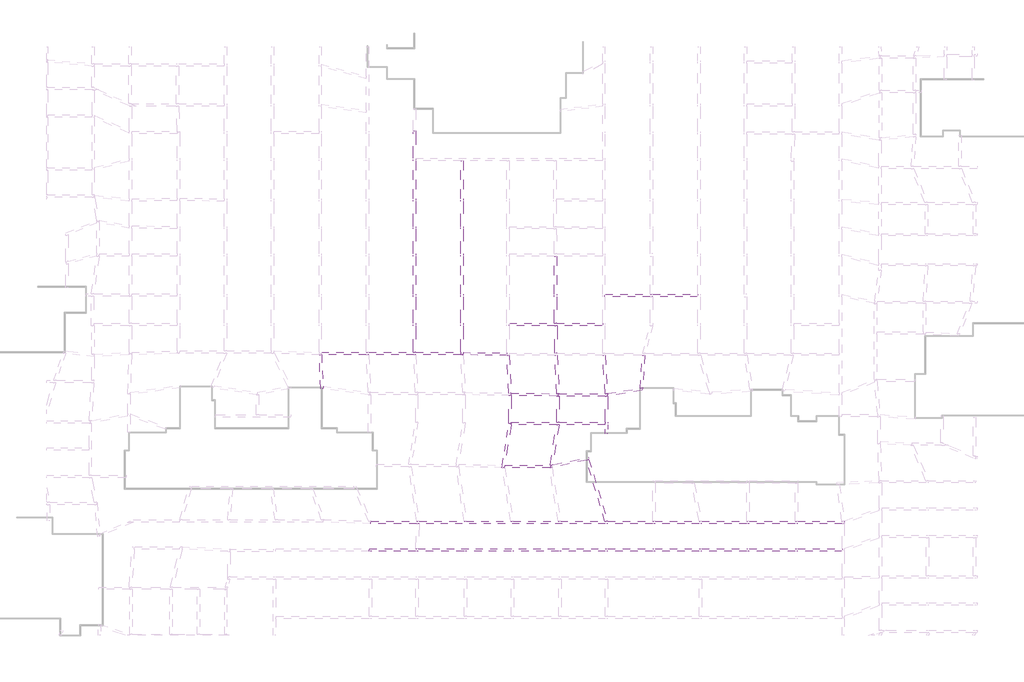
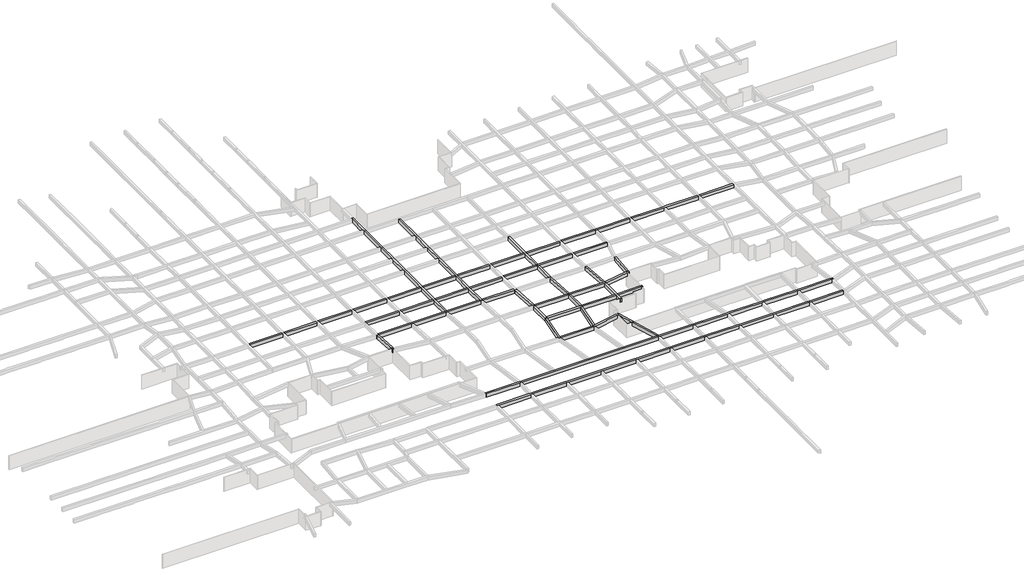
# One storey, part 21 of 45: 27 beams.
"""IFC4 building model written with IfcOpenShell, lengths in millimetres."""

from ifc_helpers import new_model, si_unit, frame, origin, place, context, project, spatial, polyline, outline, extrude, faceted_brep, element, save

model = new_model("IFC4")

# Units and contexts
model_context = context("Model", 3, world=origin())
ifc_project = project(units=[si_unit("LENGTHUNIT", "METRE", prefix="MILLI")], contexts=[model_context])

# Site, building, storey
site = spatial("IfcSite", under=ifc_project)
building = spatial("IfcBuilding", under=site)
storey = spatial("IfcBuildingStorey", under=building, Name="户型图", Elevation=0.0)

# Beams
placement = place(None, origin())
element("IfcBeam", 1, ObjectType="混凝土 - 矩形梁 : KL_beam", at=placement, inside=storey, context=model_context, shape_type="Brep", body=[
    faceted_brep([(-45810.5958048, 7704.0007632, 3300.0), (-45411.0008038, 7704.0007632, 3300.0), (-45410.5958048, 7704.0007632, 3300.0), (-45410.5958048, 7704.0007632, 2500.0), (-45411.0008038, 7704.0007632, 2500.0), (-45810.5958048, 7704.0007632, 2500.0), (-45810.5958048, 7600.318112, 3300.0), (-45810.5958048, 7200.318112, 3300.0), (-45810.5958048, 3119.5822838, 3300.0), (-45810.5958048, 2719.5822838, 3300.0), (-45810.5958048, -3551.5199121, 3300.0), (-45810.5958048, -3951.5199121, 3300.0), (-45810.5958048, -8106.533538, 3300.0), (-45810.5958048, -8506.533538, 3300.0), (-45810.5958048, -12606.533538, 3300.0), (-45810.5958048, -13006.533538, 3300.0), (-45810.5958048, -19266.2432363, 3300.0), (-45810.5958048, -19666.2432363, 3300.0), (-45810.5958048, -24066.2432363, 3300.0), (-45810.5958048, -24466.2432363, 3300.0), (-45810.5958048, -28866.2296815, 3300.0), (-45410.5958048, -28866.2296815, 3300.0), (-45410.5958048, -24466.2432363, 3300.0), (-45410.5958048, -24066.2432363, 3300.0), (-45410.5958048, -19666.2432363, 3300.0), (-45410.5958048, -19266.2432363, 3300.0), (-45410.5958048, -13006.533538, 3300.0), (-45410.5958048, -12606.533538, 3300.0), (-45410.5958048, -8506.533538, 3300.0), (-45410.5958048, -8106.533538, 3300.0), (-45410.5958048, -3951.5199121, 3300.0), (-45410.5958048, -3551.5199121, 3300.0), (-45410.5958048, 2719.5822838, 3300.0), (-45410.5958048, 3119.5822838, 3300.0), (-45410.5958048, -28866.2296815, 2500.0), (-45410.5958048, -24466.2432363, 2500.0), (-45410.5958048, -24066.2432363, 2500.0), (-45410.5958048, -19666.2432363, 2500.0), (-45410.5958048, -19266.2432363, 2500.0), (-45410.5958048, -13006.533538, 2500.0), (-45410.5958048, -12606.533538, 2500.0), (-45410.5958048, -8506.533538, 2500.0), (-45410.5958048, -8106.533538, 2500.0), (-45410.5958048, -3951.5199121, 2500.0), (-45410.5958048, -3551.5199121, 2500.0), (-45410.5958048, 2719.5822838, 2500.0), (-45410.5958048, 3119.5822838, 2500.0), (-45810.5958048, -28866.2296815, 2500.0), (-45810.5958048, -24466.2432363, 2500.0), (-45810.5958048, -24066.2432363, 2500.0), (-45810.5958048, -19666.2432363, 2500.0), (-45810.5958048, -19266.2432363, 2500.0), (-45810.5958048, -13006.533538, 2500.0), (-45810.5958048, -12606.533538, 2500.0), (-45810.5958048, -8506.533538, 2500.0), (-45810.5958048, -8106.533538, 2500.0), (-45810.5958048, -3951.5199121, 2500.0), (-45810.5958048, -3551.5199121, 2500.0), (-45810.5958048, 2719.5822838, 2500.0), (-45810.5958048, 3119.5822838, 2500.0), (-45810.5958048, 7200.318112, 2500.0), (-45810.5958048, 7600.318112, 2500.0)], [[[0, 1, 2, 3, 4, 5]], [[2, 1, 0, 6, 7, 8, 9, 10, 11, 12, 13, 14, 15, 16, 17, 18, 19, 20, 21, 22, 23, 24, 25, 26, 27, 28, 29, 30, 31, 32, 33]], [[3, 2, 33, 32, 31, 30, 29, 28, 27, 26, 25, 24, 23, 22, 21, 34, 35, 36, 37, 38, 39, 40, 41, 42, 43, 44, 45, 46]], [[5, 4, 3, 46, 45, 44, 43, 42, 41, 40, 39, 38, 37, 36, 35, 34, 47, 48, 49, 50, 51, 52, 53, 54, 55, 56, 57, 58, 59, 60, 61]], [[0, 5, 61, 60, 59, 58, 57, 56, 55, 54, 53, 52, 51, 50, 49, 48, 47, 20, 19, 18, 17, 16, 15, 14, 13, 12, 11, 10, 9, 8, 7, 6]], [[21, 20, 47, 34]]]),
])
element("IfcBeam", 2, ObjectType="混凝土 - 矩形梁 : KL_beam", at=placement, inside=storey, context=model_context, shape_type="Brep", body=[
    faceted_brep([(-38013.9760147, -29266.2296815, 3300.0), (-38003.6741425, -29266.2296815, 3300.0), (-37783.4522617, -29266.2296815, 3300.0), (-37613.9760147, -29266.2296815, 3300.0), (-37613.9760147, -28868.360722, 3300.0), (-37613.9760147, -24466.2432363, 3300.0), (-37613.9760147, -24066.2432363, 3300.0), (-37613.9760147, -19666.2432363, 3300.0), (-37613.9760147, -19266.2432363, 3300.0), (-37613.9760147, -13006.533538, 3300.0), (-37613.9760147, -12606.533538, 3300.0), (-37613.9760147, -8506.533538, 3300.0), (-37613.9760147, -8106.533538, 3300.0), (-37613.9760147, -3951.5199121, 3300.0), (-37613.9760147, -3551.5199121, 3300.0), (-37613.9760147, 2719.5822838, 3300.0), (-38013.9760147, 2719.5822838, 3300.0), (-38013.9760147, -3551.5199121, 3300.0), (-38013.9760147, -3951.5199121, 3300.0), (-38013.9760147, -8106.533538, 3300.0), (-38013.9760147, -8506.533538, 3300.0), (-38013.9760147, -12606.533538, 3300.0), (-38013.9760147, -13006.533538, 3300.0), (-38013.9760147, -19266.2432363, 3300.0), (-38013.9760147, -19666.2432363, 3300.0), (-38013.9760147, -24066.2432363, 3300.0), (-38013.9760147, -24466.2432363, 3300.0), (-38013.9760147, -28866.2296815, 3300.0), (-38013.9760147, -29266.2296815, 2500.0), (-38013.9760147, 2719.5822838, 2500.0), (-38013.9760147, -3551.5199121, 2500.0), (-38013.9760147, -3951.5199121, 2500.0), (-38013.9760147, -8106.533538, 2500.0), (-38013.9760147, -8506.533538, 2500.0), (-38013.9760147, -12606.533538, 2500.0), (-38013.9760147, -13006.533538, 2500.0), (-38013.9760147, -19266.2432363, 2500.0), (-38013.9760147, -19666.2432363, 2500.0), (-38013.9760147, -24066.2432363, 2500.0), (-38013.9760147, -24466.2432363, 2500.0), (-38013.9760147, -28866.2296815, 2500.0), (-37613.9760147, -29266.2296815, 2500.0), (-37783.4522617, -29266.2296815, 2500.0), (-38003.6741425, -29266.2296815, 2500.0), (-37613.9760147, 2719.5822838, 2500.0), (-37613.9760147, -3551.5199121, 2500.0), (-37613.9760147, -3951.5199121, 2500.0), (-37613.9760147, -8106.533538, 2500.0), (-37613.9760147, -8506.533538, 2500.0), (-37613.9760147, -12606.533538, 2500.0), (-37613.9760147, -13006.533538, 2500.0), (-37613.9760147, -19266.2432363, 2500.0), (-37613.9760147, -19666.2432363, 2500.0), (-37613.9760147, -24066.2432363, 2500.0), (-37613.9760147, -24466.2432363, 2500.0), (-37613.9760147, -28868.360722, 2500.0)], [[[0, 1, 2, 3, 4, 5, 6, 7, 8, 9, 10, 11, 12, 13, 14, 15, 16, 17, 18, 19, 20, 21, 22, 23, 24, 25, 26, 27]], [[28, 0, 27, 26, 25, 24, 23, 22, 21, 20, 19, 18, 17, 16, 29, 30, 31, 32, 33, 34, 35, 36, 37, 38, 39, 40]], [[41, 42, 43, 28, 40, 39, 38, 37, 36, 35, 34, 33, 32, 31, 30, 29, 44, 45, 46, 47, 48, 49, 50, 51, 52, 53, 54, 55]], [[3, 41, 55, 54, 53, 52, 51, 50, 49, 48, 47, 46, 45, 44, 15, 14, 13, 12, 11, 10, 9, 8, 7, 6, 5, 4]], [[16, 15, 44, 29]], [[3, 2, 1, 0, 28, 43, 42, 41]]]),
])
element("IfcBeam", 3, ObjectType="混凝土 - 矩形梁 : KL_beam", at=placement, inside=storey, context=model_context, shape_type="Brep", body=[
    faceted_brep([(-22569.0047968, -24066.2432363, 2500.0), (-22569.0047968, -24066.2432363, 3300.0), (-22569.0047968, -19666.2432363, 3300.0), (-22569.0047968, -19266.2432363, 3300.0), (-22569.0047968, -13006.533538, 3300.0), (-22569.0047968, -13006.533538, 2500.0), (-22569.0047968, -19266.2432363, 2500.0), (-22569.0047968, -19666.2432363, 2500.0), (-22169.0047968, -24066.2432363, 2500.0), (-22169.0047968, -24066.2432363, 3300.0), (-22169.0047968, -13006.533538, 3300.0), (-22169.0047968, -13006.533538, 2500.0), (-22169.0047968, -19666.2432363, 3300.0), (-22169.0047968, -19266.2432363, 3300.0), (-22169.0047968, -19266.2432363, 2500.0), (-22169.0047968, -19666.2432363, 2500.0)], [[[0, 1, 2, 3, 4, 5, 6, 7]], [[1, 0, 8, 9]], [[10, 11, 5, 4]], [[10, 4, 3, 2, 1, 9, 12, 13]], [[5, 11, 14, 15, 8, 0, 7, 6]], [[11, 10, 13, 12, 9, 8, 15, 14]]]),
])
element("IfcBeam", 4, ObjectType="混凝土 - 矩形梁 : KL_beam", at=placement, inside=storey, context=model_context, shape_type="Brep", body=[
    faceted_brep([(-60985.2176693, -24066.2432363, 3300.0), (-60985.2176693, -24466.2432363, 3300.0), (-53571.0209029, -24466.2432363, 3300.0), (-53571.0209029, -24066.2432363, 3300.0), (-60985.2176693, -24466.2432363, 2500.0), (-53571.0209029, -24466.2432363, 2500.0), (-60985.2176693, -24066.2432363, 2500.0), (-53571.0209029, -24066.2432363, 2500.0)], [[[0, 1, 2, 3]], [[1, 4, 5, 2]], [[4, 6, 7, 5]], [[6, 0, 3, 7]], [[1, 0, 6, 4]], [[3, 2, 5, 7]]]),
    faceted_brep([(-6728.2347705, -24066.2432363, 3300.0), (-6728.2347705, -24466.2432363, 3300.0), (-6728.2347705, -24466.2432363, 2500.0), (-6728.2347705, -24066.2432363, 2500.0), (-14228.2347705, -24466.2432363, 3300.0), (-14228.2347705, -24066.2432363, 3300.0), (-14228.2347705, -24066.2432363, 2500.0), (-14228.2347705, -24466.2432363, 2500.0), (-6789.3712945, -24466.2432363, 3300.0), (-6789.3712945, -24466.2432363, 2500.0)], [[[0, 1, 2, 3]], [[4, 5, 6, 7]], [[1, 0, 5, 4, 8]], [[2, 1, 8, 4, 7, 9]], [[3, 2, 9, 7, 6]], [[0, 3, 6, 5]]]),
    faceted_brep([(-53171.0209029, -24466.2432363, 3300.0), (-53171.0209029, -24066.2432363, 3300.0), (-53171.0209029, -24066.2432363, 2500.0), (-53171.0209029, -24466.2432363, 2500.0), (-45810.5958048, -24066.2432363, 3300.0), (-45810.5958048, -24466.2432363, 3300.0), (-45810.5958048, -24466.2432363, 2500.0), (-45810.5958048, -24066.2432363, 2500.0)], [[[0, 1, 2, 3]], [[4, 5, 6, 7]], [[1, 0, 5, 4]], [[0, 3, 6, 5]], [[3, 2, 7, 6]], [[2, 1, 4, 7]]]),
    faceted_brep([(-45410.5958048, -24066.2432363, 3300.0), (-45410.5958048, -24466.2432363, 3300.0), (-38013.9760147, -24466.2432363, 3300.0), (-38013.9760147, -24066.2432363, 3300.0), (-45410.5958048, -24466.2432363, 2500.0), (-38013.9760147, -24466.2432363, 2500.0), (-45410.5958048, -24066.2432363, 2500.0), (-38013.9760147, -24066.2432363, 2500.0)], [[[0, 1, 2, 3]], [[1, 4, 5, 2]], [[4, 6, 7, 5]], [[6, 0, 3, 7]], [[1, 0, 6, 4]], [[3, 2, 5, 7]]]),
    faceted_brep([(-37613.9760147, -24466.2432363, 3300.0), (-37613.9760147, -24066.2432363, 3300.0), (-37613.9760147, -24066.2432363, 2500.0), (-37613.9760147, -24466.2432363, 2500.0), (-30405.4489038, -24066.2432363, 3300.0), (-30405.4489038, -24466.2432363, 3300.0), (-30405.4489038, -24466.2432363, 2500.0), (-30405.4489038, -24066.2432363, 2500.0)], [[[0, 1, 2, 3]], [[4, 5, 6, 7]], [[1, 0, 5, 4]], [[0, 3, 6, 5]], [[3, 2, 7, 6]], [[2, 1, 4, 7]]]),
    faceted_brep([(-30005.4489038, -24066.2432363, 3300.0), (-30005.4489038, -24466.2432363, 3300.0), (-22523.4502387, -24466.2432363, 3300.0), (-22123.4502387, -24466.2432363, 3300.0), (-14628.2347705, -24466.2432363, 3300.0), (-14628.2347705, -24066.2432363, 3300.0), (-22169.0047968, -24066.2432363, 3300.0), (-22569.0047968, -24066.2432363, 3300.0), (-30005.4489038, -24466.2432363, 2500.0), (-22523.4502387, -24466.2432363, 2500.0), (-22123.4502387, -24466.2432363, 2500.0), (-14628.2347705, -24466.2432363, 2500.0), (-30005.4489038, -24066.2432363, 2500.0), (-22569.0047968, -24066.2432363, 2500.0), (-22169.0047968, -24066.2432363, 2500.0), (-14628.2347705, -24066.2432363, 2500.0)], [[[0, 1, 2, 3, 4, 5, 6, 7]], [[1, 8, 9, 10, 11, 4, 3, 2]], [[8, 12, 13, 14, 15, 11, 10, 9]], [[12, 0, 7, 6, 5, 15, 14, 13]], [[1, 0, 12, 8]], [[5, 4, 11, 15]]]),
])
element("IfcBeam", 5, ObjectType="混凝土 - 矩形梁 : KL_beam", at=placement, inside=storey, context=model_context, shape_type="Brep", body=[
    faceted_brep([(24442.7166646, -19666.2432363, 3300.0), (24442.7166646, -19266.2432363, 3300.0), (16905.3597604, -19266.2432363, 3300.0), (16905.3597604, -19666.2432363, 3300.0), (24442.7166646, -19266.2432363, 2500.0), (16905.3597604, -19266.2432363, 2500.0), (24442.7166646, -19666.2432363, 2500.0), (16905.3597604, -19666.2432363, 2500.0)], [[[0, 1, 2, 3]], [[1, 4, 5, 2]], [[4, 6, 7, 5]], [[6, 0, 3, 7]], [[1, 0, 6, 4]], [[3, 2, 5, 7]]]),
    faceted_brep([(-84386.4058027, -19666.2432363, 3300.0), (-84386.4058027, -19266.2432363, 3300.0), (-84386.4058027, -19266.2432363, 2500.0), (-84386.4058027, -19666.2432363, 2500.0), (-76974.0592951, -19266.2432363, 3300.0), (-76974.0592951, -19666.2432363, 3300.0), (-76974.0592951, -19666.2432363, 2500.0), (-76974.0592951, -19266.2432363, 2500.0)], [[[0, 1, 2, 3]], [[4, 5, 6, 7]], [[1, 0, 5, 4]], [[2, 1, 4, 7]], [[3, 2, 7, 6]], [[0, 3, 6, 5]]]),
    faceted_brep([(-76574.0592951, -19666.2432363, 3300.0), (-76574.0592951, -19266.2432363, 3300.0), (-76574.0592951, -19266.2432363, 2500.0), (-76574.0592951, -19666.2432363, 2500.0), (-69259.410716, -19266.2432363, 3300.0), (-69259.410716, -19666.2432363, 3300.0), (-69259.410716, -19666.2432363, 2500.0), (-69259.410716, -19266.2432363, 2500.0)], [[[0, 1, 2, 3]], [[4, 5, 6, 7]], [[1, 0, 5, 4]], [[2, 1, 4, 7]], [[3, 2, 7, 6]], [[0, 3, 6, 5]]]),
    faceted_brep([(-68859.410716, -19666.2432363, 3300.0), (-68859.410716, -19266.2432363, 3300.0), (-68859.410716, -19266.2432363, 2500.0), (-68859.410716, -19666.2432363, 2500.0), (-61385.2176693, -19266.2432363, 3300.0), (-61385.2176693, -19666.2432363, 3300.0), (-61385.2176693, -19666.2432363, 2500.0), (-61385.2176693, -19266.2432363, 2500.0)], [[[0, 1, 2, 3]], [[4, 5, 6, 7]], [[1, 0, 5, 4]], [[2, 1, 4, 7]], [[3, 2, 7, 6]], [[0, 3, 6, 5]]]),
    faceted_brep([(-60985.2176693, -19666.2432363, 3300.0), (-60985.2176693, -19266.2432363, 3300.0), (-60985.2176693, -19266.2432363, 2500.0), (-60985.2176693, -19666.2432363, 2500.0), (-53571.0209029, -19266.2432363, 3300.0), (-53571.0209029, -19666.2432363, 3300.0), (-53571.0209029, -19666.2432363, 2500.0), (-53571.0209029, -19266.2432363, 2500.0)], [[[0, 1, 2, 3]], [[4, 5, 6, 7]], [[1, 0, 5, 4]], [[2, 1, 4, 7]], [[3, 2, 7, 6]], [[0, 3, 6, 5]]]),
    faceted_brep([(-53171.0209029, -19666.2432363, 3300.0), (-53171.0209029, -19266.2432363, 3300.0), (-53171.0209029, -19266.2432363, 2500.0), (-53171.0209029, -19666.2432363, 2500.0), (-45810.5958048, -19266.2432363, 3300.0), (-45810.5958048, -19666.2432363, 3300.0), (-45810.5958048, -19666.2432363, 2500.0), (-45810.5958048, -19266.2432363, 2500.0)], [[[0, 1, 2, 3]], [[4, 5, 6, 7]], [[1, 0, 5, 4]], [[2, 1, 4, 7]], [[3, 2, 7, 6]], [[0, 3, 6, 5]]]),
    faceted_brep([(-45410.5958048, -19666.2432363, 3300.0), (-45410.5958048, -19266.2432363, 3300.0), (-45410.5958048, -19266.2432363, 2500.0), (-45410.5958048, -19666.2432363, 2500.0), (-38013.9760147, -19266.2432363, 3300.0), (-38013.9760147, -19666.2432363, 3300.0), (-38013.9760147, -19666.2432363, 2500.0), (-38013.9760147, -19266.2432363, 2500.0)], [[[0, 1, 2, 3]], [[4, 5, 6, 7]], [[1, 0, 5, 4]], [[2, 1, 4, 7]], [[3, 2, 7, 6]], [[0, 3, 6, 5]]]),
    faceted_brep([(-37613.9760147, -19666.2432363, 3300.0), (-37613.9760147, -19266.2432363, 3300.0), (-37613.9760147, -19266.2432363, 2500.0), (-37613.9760147, -19666.2432363, 2500.0), (-30405.4489038, -19266.2432363, 3300.0), (-30405.4489038, -19666.2432363, 3300.0), (-30405.4489038, -19666.2432363, 2500.0), (-30405.4489038, -19266.2432363, 2500.0)], [[[0, 1, 2, 3]], [[4, 5, 6, 7]], [[1, 0, 5, 4]], [[2, 1, 4, 7]], [[3, 2, 7, 6]], [[0, 3, 6, 5]]]),
    faceted_brep([(-30005.4489038, -19666.2432363, 3300.0), (-30005.4489038, -19266.2432363, 3300.0), (-30005.4489038, -19266.2432363, 2500.0), (-30005.4489038, -19666.2432363, 2500.0), (-22569.0047968, -19266.2432363, 3300.0), (-22569.0047968, -19666.2432363, 3300.0), (-22569.0047968, -19666.2432363, 2500.0), (-22569.0047968, -19266.2432363, 2500.0)], [[[0, 1, 2, 3]], [[4, 5, 6, 7]], [[1, 0, 5, 4]], [[2, 1, 4, 7]], [[3, 2, 7, 6]], [[0, 3, 6, 5]]]),
    faceted_brep([(-22169.0047968, -19666.2432363, 3300.0), (-22169.0047968, -19266.2432363, 3300.0), (-22169.0047968, -19266.2432363, 2500.0), (-22169.0047968, -19666.2432363, 2500.0), (-14628.2347705, -19266.2432363, 3300.0), (-14628.2347705, -19666.2432363, 3300.0), (-14628.2347705, -19666.2432363, 2500.0), (-14628.2347705, -19266.2432363, 2500.0)], [[[0, 1, 2, 3]], [[4, 5, 6, 7]], [[1, 0, 5, 4]], [[2, 1, 4, 7]], [[3, 2, 7, 6]], [[0, 3, 6, 5]]]),
    faceted_brep([(-14228.2347705, -19666.2432363, 3300.0), (-14228.2347705, -19266.2432363, 3300.0), (-14228.2347705, -19266.2432363, 2500.0), (-14228.2347705, -19666.2432363, 2500.0), (1071.7652295, -19266.2432363, 3300.0), (1071.7652295, -19666.2432363, 3300.0), (1071.7652295, -19666.2432363, 2500.0), (1071.7652295, -19266.2432363, 2500.0), (-6728.2347705, -19666.2432363, 3300.0), (-6328.2347705, -19666.2432363, 3300.0), (-6328.2347705, -19266.2432363, 3300.0), (-6728.2347705, -19266.2432363, 3300.0), (-6328.2347705, -19266.2432363, 2500.0), (-6728.2347705, -19266.2432363, 2500.0), (-6328.2347705, -19666.2432363, 2500.0), (-6728.2347705, -19666.2432363, 2500.0)], [[[0, 1, 2, 3]], [[4, 5, 6, 7]], [[1, 0, 8, 9, 5, 4, 10, 11]], [[2, 1, 11, 10, 4, 7, 12, 13]], [[3, 2, 13, 12, 7, 6, 14, 15]], [[0, 3, 15, 14, 6, 5, 9, 8]]]),
    faceted_brep([(1471.7652295, -19666.2432363, 3300.0), (1471.7652295, -19266.2432363, 3300.0), (1471.7652295, -19266.2432363, 2500.0), (1471.7652295, -19666.2432363, 2500.0), (16505.3597604, -19266.2432363, 3300.0), (16505.3597604, -19666.2432363, 3300.0), (16505.3597604, -19666.2432363, 2500.0), (16505.3597604, -19266.2432363, 2500.0), (8769.3873949, -19666.2432363, 3300.0), (9169.3873949, -19666.2432363, 3300.0), (9169.3873949, -19266.2432363, 3300.0), (8769.3873949, -19266.2432363, 3300.0), (9169.3873949, -19266.2432363, 2500.0), (8769.3873949, -19266.2432363, 2500.0), (9169.3873949, -19666.2432363, 2500.0), (8769.3873949, -19666.2432363, 2500.0)], [[[0, 1, 2, 3]], [[4, 5, 6, 7]], [[1, 0, 8, 9, 5, 4, 10, 11]], [[2, 1, 11, 10, 4, 7, 12, 13]], [[3, 2, 13, 12, 7, 6, 14, 15]], [[0, 3, 15, 14, 6, 5, 9, 8]]]),
])
element("IfcBeam", 6, ObjectType="混凝土 - 矩形梁 : KL_beam", at=placement, inside=storey, context=model_context, shape_type="Brep", body=[
    faceted_brep([(-38013.9760147, -29266.2296815, 3300.0), (-38013.9760147, -28866.2296815, 3300.0), (-45410.5958048, -28866.2296815, 3300.0), (-45810.5958048, -28866.2296815, 3300.0), (-53171.0209029, -28866.2296815, 3300.0), (-53571.0209029, -28866.2296815, 3300.0), (-60985.2176693, -28866.2296815, 3300.0), (-60985.2176693, -29259.522509, 3300.0), (-60985.2176693, -29266.2296815, 3300.0), (-60974.4623546, -29266.2296815, 3300.0), (-53560.8025287, -29266.2296815, 3300.0), (-53160.2535903, -29266.2296815, 3300.0), (-45800.3887182, -29266.2296815, 3300.0), (-45399.8397798, -29266.2296815, 3300.0), (-38013.9760147, -29266.2296815, 2500.0), (-60985.2176693, -29266.2296815, 2500.0), (-60974.4623546, -29266.2296815, 2500.0), (-53560.8025287, -29266.2296815, 2500.0), (-53160.2535903, -29266.2296815, 2500.0), (-45800.3887182, -29266.2296815, 2500.0), (-45399.8397798, -29266.2296815, 2500.0), (-38013.9760147, -28866.2296815, 2500.0), (-60985.2176693, -29259.522509, 2500.0), (-60985.2176693, -28866.2296815, 2500.0), (-53571.0209029, -28866.2296815, 2500.0), (-53171.0209029, -28866.2296815, 2500.0), (-45810.5958048, -28866.2296815, 2500.0), (-45410.5958048, -28866.2296815, 2500.0)], [[[0, 1, 2, 3, 4, 5, 6, 7, 8, 9, 10, 11, 12, 13]], [[14, 0, 13, 12, 11, 10, 9, 8, 15, 16, 17, 18, 19, 20]], [[21, 14, 20, 19, 18, 17, 16, 15, 22, 23, 24, 25, 26, 27]], [[1, 21, 27, 26, 25, 24, 23, 6, 5, 4, 3, 2]], [[1, 0, 14, 21]], [[15, 8, 7, 6, 23, 22]]]),
    faceted_brep([(-61375.011293, -29266.2296815, 2500.0), (-61375.011293, -29266.2296815, 3300.0), (-61375.3451123, -29259.8600307, 3300.0), (-61375.3451123, -29259.8600307, 2500.0), (-61189.0319378, -29266.2296815, 3300.0), (-61189.0319378, -29266.2296815, 2500.0)], [[[0, 1, 2, 3]], [[2, 4, 5, 3]], [[1, 4, 2]], [[1, 0, 5, 4]], [[5, 0, 3]]]),
])
element("IfcBeam", 7, ObjectType="混凝土 - 矩形梁 : KL_beam", at=placement, inside=storey, context=model_context, shape_type="Brep", body=[
    faceted_brep([(-30005.4489038, -29365.5283832, 3300.0), (-30005.4489038, -29362.9587641, 3300.0), (-30005.4489038, -29360.4217409, 3300.0), (-30405.4489038, -29360.4217409, 3300.0), (-30395.4415902, -29360.5495003, 3300.0), (-30005.4489038, -29365.5283832, 2500.0), (-37603.004472, -29268.5333873, 3300.0), (-37783.4522617, -29266.2296815, 3300.0), (-37783.4522617, -29266.2296815, 2500.0), (-37603.004472, -29268.5333873, 2500.0), (-30405.4489038, -29360.4217409, 2500.0), (-30395.4415902, -29360.5495003, 2500.0), (-30005.4489038, -29360.4217409, 2500.0), (-30005.4489038, -29362.9587641, 2500.0), (-30405.4489038, -28960.389145, 3300.0), (-30405.4489038, -28960.389145, 2500.0), (-37613.9760147, -28868.360722, 2500.0), (-37613.9760147, -28868.360722, 3300.0), (-37613.9760147, -29266.2296815, 3300.0), (-37613.9760147, -29266.2296815, 2500.0)], [[[0, 1, 2, 3, 4]], [[5, 0, 4, 3, 6, 7, 8, 9, 10, 11]], [[12, 13, 5, 11, 10]], [[14, 15, 16, 17]], [[0, 5, 13, 12, 2, 1]], [[3, 10, 15, 14]], [[10, 3, 2, 12]], [[3, 14, 17, 18, 7, 6]], [[15, 10, 9, 8, 19, 16]], [[19, 18, 17, 16]], [[18, 19, 8, 7]]]),
])
element("IfcBeam", 8, ObjectType="混凝土 - 矩形梁 : KL_beam", at=placement, inside=storey, context=model_context, shape_type="Brep", body=[
    faceted_brep([(-21973.5605003, -36064.095945, 3300.0), (-21971.0072832, -35664.095945, 3300.0), (-22183.1652198, -35661.3874083, 3300.0), (-29669.6887336, -35565.8099149, 3300.0), (-29648.7098773, -35966.1103396, 3300.0), (-22172.2672463, -36061.5591344, 3300.0), (-21973.5605003, -36064.095945, 2500.0), (-29648.7098773, -35966.1103396, 2500.0), (-22172.2672463, -36061.5591344, 2500.0), (-21971.0072832, -35664.095945, 2500.0), (-29669.6887336, -35565.8099149, 2500.0), (-22183.1652198, -35661.3874083, 2500.0)], [[[0, 1, 2, 3, 4, 5]], [[6, 0, 5, 4, 7, 8]], [[9, 6, 8, 7, 10, 11]], [[1, 9, 11, 10, 3, 2]], [[1, 0, 6, 9]], [[4, 3, 10, 7]]]),
])
element("IfcBeam", 9, ObjectType="混凝土 - 矩形梁 : KL_beam", at=placement, inside=storey, context=model_context, shape_type="Brep", body=[
    faceted_brep([(-13785.4296353, -35664.095945, 3300.0), (-14186.3544768, -35664.095945, 3300.0), (-21782.474333, -35664.095945, 3300.0), (-21971.0072832, -35664.095945, 3300.0), (-21973.5605003, -36064.095945, 3300.0), (-21772.2672463, -36064.095945, 3300.0), (-14172.2838918, -36064.095945, 3300.0), (-13785.4296353, -36064.095945, 3300.0), (-21973.5605003, -36064.095945, 2500.0), (-21772.2672463, -36064.095945, 2500.0), (-14172.2838918, -36064.095945, 2500.0), (-13785.4296353, -36064.095945, 2500.0), (-21971.0072832, -35664.095945, 2500.0), (-21782.474333, -35664.095945, 2500.0), (-14186.3544768, -35664.095945, 2500.0), (-13785.4296353, -35664.095945, 2500.0)], [[[0, 1, 2, 3, 4, 5, 6, 7]], [[7, 6, 5, 4, 8, 9, 10, 11]], [[11, 10, 9, 8, 12, 13, 14, 15]], [[3, 2, 1, 0, 15, 14, 13, 12]], [[3, 12, 8, 4]], [[0, 7, 11, 15]]]),
])
element("IfcBeam", 10, ObjectType="混凝土 - 矩形梁 : KL_beam", at=placement, inside=storey, context=model_context, shape_type="Brep", body=[
    faceted_brep([(-13785.4296353, -36064.095945, 3300.0), (-13772.2838918, -36064.095945, 3300.0), (-13758.2133067, -36064.095945, 3300.0), (-13760.3278463, -36033.0184306, 3300.0), (-13772.2838918, -35857.2997197, 3300.0), (-13785.4296353, -35664.095945, 3300.0), (-14186.3544768, -35664.095945, 2500.0), (-14186.3544768, -35664.095945, 3300.0), (-14615.089027, -29362.9587641, 3300.0), (-14615.089027, -29362.9587641, 2500.0), (-13758.2133067, -36064.095945, 2500.0), (-13772.2838918, -36064.095945, 2500.0), (-13785.4296353, -36064.095945, 2500.0), (-13785.4296353, -35664.095945, 2500.0), (-13772.2838918, -35857.2997197, 2500.0), (-13760.3278463, -36033.0184306, 2500.0), (-13787.5896402, -35632.3502242, 2500.0), (-14214.1641855, -29362.9587641, 2500.0), (-14214.1641855, -29362.9587641, 3300.0), (-13787.5896402, -35632.3502242, 3300.0)], [[[0, 1, 2, 3, 4, 5]], [[6, 7, 8, 9]], [[10, 11, 12, 13, 14, 15]], [[2, 10, 15, 14, 13, 16, 17, 18, 19, 5, 4, 3]], [[10, 2, 1, 0, 12, 11]], [[13, 5, 7, 6]], [[5, 13, 12, 0]], [[7, 5, 19, 18, 8]], [[13, 6, 9, 17, 16]], [[9, 8, 18, 17]]]),
])
element("IfcBeam", 11, ObjectType="混凝土 - 矩形梁 : KL_beam", at=placement, inside=storey, context=model_context, shape_type="Brep", body=[
    faceted_brep([(-13772.2838918, -42264.095945, 3300.0), (-14172.2838918, -42264.095945, 3300.0), (-14172.2838918, -42264.095945, 2500.0), (-13772.2838918, -42264.095945, 2500.0), (-13772.2838918, -40763.4015903, 3300.0), (-13772.2838918, -40363.4015903, 3300.0), (-13772.2838918, -36064.095945, 3300.0), (-13785.4296353, -36064.095945, 3300.0), (-14172.2838918, -36064.095945, 3300.0), (-14172.2838918, -40363.4015903, 3300.0), (-14172.2838918, -40763.4015903, 3300.0), (-14172.2838918, -36064.095945, 2500.0), (-14172.2838918, -40363.4015903, 2500.0), (-14172.2838918, -40763.4015903, 2500.0), (-13785.4296353, -36064.095945, 2500.0), (-13772.2838918, -36064.095945, 2500.0), (-13772.2838918, -40363.4015903, 2500.0), (-13772.2838918, -40763.4015903, 2500.0)], [[[0, 1, 2, 3]], [[1, 0, 4, 5, 6, 7, 8, 9, 10]], [[2, 1, 10, 9, 8, 11, 12, 13]], [[3, 2, 13, 12, 11, 14, 15, 16, 17]], [[0, 3, 17, 16, 15, 6, 5, 4]], [[11, 8, 7, 6, 15, 14]]]),
    faceted_brep([(-13772.2838918, -35629.9260318, 3300.0), (-13772.2838918, -35629.9260318, 2500.0), (-13787.5896402, -35632.3502242, 2500.0), (-13787.5896402, -35632.3502242, 3300.0), (-13772.2838918, -35857.2997197, 3300.0), (-13785.4296353, -35664.095945, 3300.0), (-13785.4296353, -35664.095945, 2500.0), (-13772.2838918, -35857.2997197, 2500.0)], [[[0, 1, 2, 3]], [[4, 5, 3, 2, 6, 7]], [[4, 0, 3, 5]], [[2, 1, 7, 6]], [[1, 0, 4, 7]]]),
])
element("IfcBeam", 12, ObjectType="混凝土 - 矩形梁 : KL_beam", at=placement, inside=storey, context=model_context, shape_type="Brep", body=[
    faceted_brep([(-29674.7949597, -35965.7773217, 3300.0), (-29659.6078619, -35965.9712094, 3300.0), (-29648.7098773, -35966.1103396, 3300.0), (-29669.6887336, -35565.8099149, 3300.0), (-30070.5058465, -35560.6928409, 2500.0), (-30070.5058465, -35560.6928409, 3300.0), (-30395.4415902, -29360.5495003, 3300.0), (-30395.4415902, -29360.5495003, 2500.0), (-29648.7098773, -35966.1103396, 2500.0), (-29659.6078619, -35965.9712094, 2500.0), (-29674.7949597, -35965.7773217, 2500.0), (-29669.6887336, -35565.8099149, 2500.0), (-29994.7663876, -29362.9587641, 2500.0), (-29994.7663876, -29362.9587641, 3300.0), (-30005.4489038, -29362.9587641, 3300.0), (-30005.4489038, -29365.5283832, 3300.0), (-30206.7255123, -29362.9587641, 3300.0), (-30206.7255123, -29362.9587641, 2500.0), (-30005.4489038, -29365.5283832, 2500.0), (-30005.4489038, -29362.9587641, 2500.0)], [[[0, 1, 2, 3]], [[4, 5, 6, 7]], [[8, 9, 10, 11]], [[2, 8, 11, 12, 13, 3]], [[8, 2, 1, 0, 10, 9]], [[11, 3, 5, 4]], [[3, 11, 10, 0]], [[5, 3, 13, 14, 15, 16, 6]], [[11, 4, 7, 17, 18, 19, 12]], [[15, 18, 17, 7, 6, 16]], [[18, 15, 14, 19]], [[13, 12, 19, 14]]]),
])
element("IfcBeam", 13, ObjectType="混凝土 - 矩形梁 : KL_beam", at=placement, inside=storey, context=model_context, shape_type="Brep", body=[
    faceted_brep([(-30059.6078619, -35960.8645671, 3300.0), (-30059.6078619, -40547.6612489, 3300.0), (-29659.6078619, -40579.1419316, 3300.0), (-29659.6078619, -40363.4015903, 3300.0), (-29659.6078619, -35965.9712094, 3300.0), (-29674.7949597, -35965.7773217, 3300.0), (-30059.6078619, -35960.8645671, 2500.0), (-30059.6078619, -40547.6612489, 2500.0), (-29674.7949597, -35965.7773217, 2500.0), (-29659.6078619, -35965.9712094, 2500.0), (-29659.6078619, -40363.4015903, 2500.0), (-29659.6078619, -40579.1419316, 2500.0)], [[[0, 1, 2, 3, 4, 5]], [[1, 0, 6, 7]], [[7, 6, 8, 9, 10, 11]], [[4, 3, 2, 11, 10, 9]], [[6, 0, 5, 4, 9, 8]], [[2, 1, 7, 11]]]),
])
element("IfcBeam", 14, ObjectType="混凝土 - 矩形梁 : KL_beam", at=placement, inside=storey, context=model_context, shape_type="Brep", body=[
    faceted_brep([(-29659.6078619, -40579.1419316, 3300.0), (-30059.6078619, -40547.6612489, 3300.0), (-31156.1548972, -47470.9867541, 3300.0), (-31219.30506, -47869.7011904, 3300.0), (-31156.9695795, -47871.0646021, 3300.0), (-30815.7171231, -47878.528531, 3300.0), (-30815.1198731, -47874.7576426, 3300.0), (-30751.7660969, -47474.7576426, 3300.0), (-29688.7917248, -40763.4015903, 3300.0), (-30059.6078619, -40547.6612489, 2500.0), (-31156.1548972, -47470.9867541, 2500.0), (-31219.30506, -47869.7011904, 2500.0), (-29659.6078619, -40579.1419316, 2500.0), (-29688.7917248, -40763.4015903, 2500.0), (-30751.7660969, -47474.7576426, 2500.0), (-30815.1198731, -47874.7576426, 2500.0), (-30815.7171231, -47878.528531, 2500.0), (-31156.9695795, -47871.0646021, 2500.0)], [[[0, 1, 2, 3, 4, 5, 6, 7, 8]], [[1, 9, 10, 11, 3, 2]], [[9, 12, 13, 14, 15, 16, 17, 11, 10]], [[12, 0, 8, 7, 6, 5, 16, 15, 14, 13]], [[0, 12, 9, 1]], [[5, 4, 3, 11, 17, 16]]]),
])
element("IfcBeam", 15, ObjectType="混凝土 - 矩形梁 : KL_beam", at=placement, inside=storey, context=model_context, shape_type="Brep", body=[
    faceted_brep([(-23206.9568572, -47474.7576426, 3300.0), (-23269.4357365, -47474.7576426, 3300.0), (-30751.7660969, -47474.7576426, 3300.0), (-30752.5669603, -47479.8140947, 3300.0), (-30815.1198731, -47874.7576426, 3300.0), (-30751.3986091, -47874.7576426, 3300.0), (-23356.7521472, -47874.7576426, 3300.0), (-23164.9151631, -47874.7576426, 3300.0), (-30815.1198731, -47874.7576426, 2500.0), (-30751.3986091, -47874.7576426, 2500.0), (-23356.7521472, -47874.7576426, 2500.0), (-23164.9151631, -47874.7576426, 2500.0), (-30752.5669603, -47479.8140947, 2500.0), (-30751.7660969, -47474.7576426, 2500.0), (-23269.4357365, -47474.7576426, 2500.0), (-23206.9568572, -47474.7576426, 2500.0)], [[[0, 1, 2, 3, 4, 5, 6, 7]], [[7, 6, 5, 4, 8, 9, 10, 11]], [[11, 10, 9, 8, 12, 13, 14, 15]], [[2, 1, 0, 15, 14, 13]], [[8, 4, 3, 2, 13, 12]], [[0, 7, 11, 15]]]),
])
element("IfcBeam", 16, ObjectType="混凝土 - 矩形梁 : KL_beam", at=placement, inside=storey, context=model_context, shape_type="Brep", body=[
    faceted_brep([(-23206.9568572, -47474.7576426, 3300.0), (-23164.9151631, -47874.7576426, 3300.0), (-22958.7081892, -47830.9269972, 3300.0), (-17259.9319767, -46619.6147198, 3300.0), (-16867.332687, -46536.1651646, 3300.0), (-16982.9097945, -46151.7955992, 3300.0), (-22852.5172455, -47399.4191774, 3300.0), (-23164.9151631, -47874.7576426, 2500.0), (-22958.7081892, -47830.9269972, 2500.0), (-17259.9319767, -46619.6147198, 2500.0), (-16867.332687, -46536.1651646, 2500.0), (-23206.9568572, -47474.7576426, 2500.0), (-22852.5172455, -47399.4191774, 2500.0), (-16982.9097945, -46151.7955992, 2500.0)], [[[0, 1, 2, 3, 4, 5, 6]], [[1, 7, 8, 9, 10, 4, 3, 2]], [[7, 11, 12, 13, 10, 9, 8]], [[11, 0, 6, 5, 13, 12]], [[0, 11, 7, 1]], [[5, 4, 10, 13]]]),
])
element("IfcBeam", 17, ObjectType="混凝土 - 矩形梁 : KL_beam", at=placement, inside=storey, context=model_context, shape_type="Brep", body=[
    faceted_brep([(-52883.6890029, -56712.697306, 3300.0), (-52890.6710288, -57112.697306, 3300.0), (-45264.9383384, -57112.697306, 3300.0), (-44864.5489511, -57112.697306, 3300.0), (-14155.9166766, -57112.697306, 3300.0), (-13755.9166766, -57112.697306, 3300.0), (-6361.9880078, -57112.697306, 3300.0), (-5961.9880078, -57112.697306, 3300.0), (1338.0119922, -57112.697306, 3300.0), (1738.0119922, -57112.697306, 3300.0), (9138.0119922, -57112.697306, 3300.0), (9538.0119922, -57112.697306, 3300.0), (17160.5867178, -57112.697306, 3300.0), (17560.5867178, -57112.697306, 3300.0), (24866.4388689, -57112.697306, 3300.0), (25266.4388689, -57112.697306, 3300.0), (25266.4388689, -57052.7388136, 3300.0), (25266.4388689, -56712.697306, 3300.0), (25031.1734727, -56712.697306, 3300.0), (24837.0666178, -56712.697306, 3300.0), (17560.5867178, -56712.697306, 3300.0), (17160.5867178, -56712.697306, 3300.0), (9538.0119922, -56712.697306, 3300.0), (9138.0119922, -56712.697306, 3300.0), (1702.8049756, -56712.697306, 3300.0), (1295.3182976, -56712.697306, 3300.0), (-5961.9880078, -56712.697306, 3300.0), (-6361.9880078, -56712.697306, 3300.0), (-13807.3241569, -56712.697306, 3300.0), (-14225.0161154, -56712.697306, 3300.0), (-21551.9739697, -56712.697306, 3300.0), (-21956.96002, -56712.697306, 3300.0), (-29351.6064819, -56712.697306, 3300.0), (-29756.5925322, -56712.697306, 3300.0), (-37070.2015905, -56712.697306, 3300.0), (-37474.2420685, -56712.697306, 3300.0), (-44882.3951564, -56712.697306, 3300.0), (-45286.4356345, -56712.697306, 3300.0), (-52756.9890549, -56712.697306, 3300.0), (-52890.6710288, -57112.697306, 2500.0), (-45264.9383384, -57112.697306, 2500.0), (-44864.5489511, -57112.697306, 2500.0), (-14155.9166766, -57112.697306, 2500.0), (-13755.9166766, -57112.697306, 2500.0), (-6361.9880078, -57112.697306, 2500.0), (-5961.9880078, -57112.697306, 2500.0), (1338.0119922, -57112.697306, 2500.0), (1738.0119922, -57112.697306, 2500.0), (9138.0119922, -57112.697306, 2500.0), (9538.0119922, -57112.697306, 2500.0), (17160.5867178, -57112.697306, 2500.0), (17560.5867178, -57112.697306, 2500.0), (24866.4388689, -57112.697306, 2500.0), (25266.4388689, -57112.697306, 2500.0), (-52883.6890029, -56712.697306, 2500.0), (-52756.9890549, -56712.697306, 2500.0), (-45286.4356345, -56712.697306, 2500.0), (-44882.3951564, -56712.697306, 2500.0), (-37474.2420685, -56712.697306, 2500.0), (-37070.2015905, -56712.697306, 2500.0), (-29756.5925322, -56712.697306, 2500.0), (-29351.6064819, -56712.697306, 2500.0), (-21956.96002, -56712.697306, 2500.0), (-21551.9739697, -56712.697306, 2500.0), (-14225.0161154, -56712.697306, 2500.0), (-13807.3241569, -56712.697306, 2500.0), (-6361.9880078, -56712.697306, 2500.0), (-5961.9880078, -56712.697306, 2500.0), (1295.3182976, -56712.697306, 2500.0), (1702.8049756, -56712.697306, 2500.0), (9138.0119922, -56712.697306, 2500.0), (9538.0119922, -56712.697306, 2500.0), (17160.5867178, -56712.697306, 2500.0), (17560.5867178, -56712.697306, 2500.0), (24837.0666178, -56712.697306, 2500.0), (25031.1734727, -56712.697306, 2500.0), (25266.4388689, -56712.697306, 2500.0), (25266.4388689, -57052.7388136, 2500.0)], [[[0, 1, 2, 3, 4, 5, 6, 7, 8, 9, 10, 11, 12, 13, 14, 15, 16, 17, 18, 19, 20, 21, 22, 23, 24, 25, 26, 27, 28, 29, 30, 31, 32, 33, 34, 35, 36, 37, 38]], [[1, 39, 40, 41, 42, 43, 44, 45, 46, 47, 48, 49, 50, 51, 52, 53, 15, 14, 13, 12, 11, 10, 9, 8, 7, 6, 5, 4, 3, 2]], [[39, 54, 55, 56, 57, 58, 59, 60, 61, 62, 63, 64, 65, 66, 67, 68, 69, 70, 71, 72, 73, 74, 75, 76, 77, 53, 52, 51, 50, 49, 48, 47, 46, 45, 44, 43, 42, 41, 40]], [[54, 0, 38, 37, 36, 35, 34, 33, 32, 31, 30, 29, 28, 27, 26, 25, 24, 23, 22, 21, 20, 19, 18, 17, 76, 75, 74, 73, 72, 71, 70, 69, 68, 67, 66, 65, 64, 63, 62, 61, 60, 59, 58, 57, 56, 55]], [[0, 54, 39, 1]], [[17, 16, 15, 53, 77, 76]]]),
])
element("IfcBeam", 18, ObjectType="混凝土 - 矩形梁 : KL_beam", at=placement, inside=storey, context=model_context, shape_type="Brep", body=[
    faceted_brep([(-53106.0296652, -61244.2645659, 3300.0), (-53106.0296652, -61644.2645659, 3300.0), (-52706.0296652, -61644.2645659, 3300.0), (-45455.9166766, -61644.2645659, 3300.0), (-45055.9166766, -61644.2645659, 3300.0), (-37455.9166766, -61644.2645659, 3300.0), (-37055.9166766, -61644.2645659, 3300.0), (-29655.9166766, -61644.2645659, 3300.0), (-29255.9166766, -61644.2645659, 3300.0), (-21855.9166766, -61644.2645659, 3300.0), (-21455.9166766, -61644.2645659, 3300.0), (-14155.9166766, -61644.2645659, 3300.0), (-13755.9166766, -61644.2645659, 3300.0), (-6361.9880078, -61644.2645659, 3300.0), (-5961.9880078, -61644.2645659, 3300.0), (1338.0119922, -61644.2645659, 3300.0), (1738.0119922, -61644.2645659, 3300.0), (9138.0119922, -61644.2645659, 3300.0), (9538.0119922, -61644.2645659, 3300.0), (17160.5867178, -61644.2645659, 3300.0), (17560.5867178, -61644.2645659, 3300.0), (24866.4388689, -61644.2645659, 3300.0), (24866.4388689, -61244.2645659, 3300.0), (17560.5867178, -61244.2645659, 3300.0), (17160.5867178, -61244.2645659, 3300.0), (9538.0119922, -61244.2645659, 3300.0), (9138.0119922, -61244.2645659, 3300.0), (1738.0119922, -61244.2645659, 3300.0), (1338.0119922, -61244.2645659, 3300.0), (-5961.9880078, -61244.2645659, 3300.0), (-6361.9880078, -61244.2645659, 3300.0), (-13755.9166766, -61244.2645659, 3300.0), (-14155.9166766, -61244.2645659, 3300.0), (-45046.8950148, -61244.2645659, 3300.0), (-45447.2844021, -61244.2645659, 3300.0), (-53106.0296652, -61644.2645659, 2500.0), (-52706.0296652, -61644.2645659, 2500.0), (-45455.9166766, -61644.2645659, 2500.0), (-45055.9166766, -61644.2645659, 2500.0), (-37455.9166766, -61644.2645659, 2500.0), (-37055.9166766, -61644.2645659, 2500.0), (-29655.9166766, -61644.2645659, 2500.0), (-29255.9166766, -61644.2645659, 2500.0), (-21855.9166766, -61644.2645659, 2500.0), (-21455.9166766, -61644.2645659, 2500.0), (-14155.9166766, -61644.2645659, 2500.0), (-13755.9166766, -61644.2645659, 2500.0), (-6361.9880078, -61644.2645659, 2500.0), (-5961.9880078, -61644.2645659, 2500.0), (1338.0119922, -61644.2645659, 2500.0), (1738.0119922, -61644.2645659, 2500.0), (9138.0119922, -61644.2645659, 2500.0), (9538.0119922, -61644.2645659, 2500.0), (17160.5867178, -61644.2645659, 2500.0), (17560.5867178, -61644.2645659, 2500.0), (24866.4388689, -61644.2645659, 2500.0), (-53106.0296652, -61244.2645659, 2500.0), (-45447.2844021, -61244.2645659, 2500.0), (-45046.8950148, -61244.2645659, 2500.0), (-14155.9166766, -61244.2645659, 2500.0), (-13755.9166766, -61244.2645659, 2500.0), (-6361.9880078, -61244.2645659, 2500.0), (-5961.9880078, -61244.2645659, 2500.0), (1338.0119922, -61244.2645659, 2500.0), (1738.0119922, -61244.2645659, 2500.0), (9138.0119922, -61244.2645659, 2500.0), (9538.0119922, -61244.2645659, 2500.0), (17160.5867178, -61244.2645659, 2500.0), (17560.5867178, -61244.2645659, 2500.0), (24866.4388689, -61244.2645659, 2500.0)], [[[0, 1, 2, 3, 4, 5, 6, 7, 8, 9, 10, 11, 12, 13, 14, 15, 16, 17, 18, 19, 20, 21, 22, 23, 24, 25, 26, 27, 28, 29, 30, 31, 32, 33, 34]], [[1, 35, 36, 37, 38, 39, 40, 41, 42, 43, 44, 45, 46, 47, 48, 49, 50, 51, 52, 53, 54, 55, 21, 20, 19, 18, 17, 16, 15, 14, 13, 12, 11, 10, 9, 8, 7, 6, 5, 4, 3, 2]], [[35, 56, 57, 58, 59, 60, 61, 62, 63, 64, 65, 66, 67, 68, 69, 55, 54, 53, 52, 51, 50, 49, 48, 47, 46, 45, 44, 43, 42, 41, 40, 39, 38, 37, 36]], [[56, 0, 34, 33, 32, 31, 30, 29, 28, 27, 26, 25, 24, 23, 22, 69, 68, 67, 66, 65, 64, 63, 62, 61, 60, 59, 58, 57]], [[1, 0, 56, 35]], [[22, 21, 55, 69]]]),
])
element("IfcBeam", 19, ObjectType="混凝土 - 矩形梁 : KL_beam", at=placement, inside=storey, context=model_context, shape_type="SweptSolid", body=[
    extrude(outline(polyline([(-17259.9319767, -46619.6147198), (-16867.332687, -46536.1651646), (-13807.3241569, -56712.697306), (-14225.0161154, -56712.697306), (-17259.9319767, -46619.6147198)])), frame((0.0, 0.0, 2500.0), z_axis=(0.0, 0.0, 1.0), x_axis=(1.0, 0.0, 0.0)), (0.0, 0.0, 1.0), 800.0),
])
element("IfcBeam", 20, ObjectType="混凝土 - 矩形梁 : KL_beam", at=placement, inside=storey, context=model_context, shape_type="Brep", body=[
    faceted_brep([(-8259.6078619, -40363.4015903, 3300.0), (-8259.6078619, -40763.4015903, 3300.0), (-8259.6078619, -40763.4015903, 2500.0), (-8259.6078619, -40363.4015903, 2500.0), (-13772.2838918, -40363.4015903, 3300.0), (-13772.2838918, -40763.4015903, 3300.0), (-13772.2838918, -40763.4015903, 2500.0), (-13772.2838918, -40363.4015903, 2500.0)], [[[0, 1, 2, 3]], [[1, 0, 4, 5]], [[2, 1, 5, 6]], [[3, 2, 6, 7]], [[0, 3, 7, 4]], [[5, 4, 7, 6]]]),
    faceted_brep([(-29659.6078619, -40579.1419316, 3300.0), (-29659.6078619, -40363.4015903, 3300.0), (-29659.6078619, -40363.4015903, 2500.0), (-29659.6078619, -40579.1419316, 2500.0), (-29688.7917248, -40763.4015903, 3300.0), (-29688.7917248, -40763.4015903, 2500.0), (-14172.2838918, -40363.4015903, 3300.0), (-14172.2838918, -40763.4015903, 3300.0), (-14172.2838918, -40763.4015903, 2500.0), (-14172.2838918, -40363.4015903, 2500.0), (-22206.4613643, -40763.4015903, 3300.0), (-21801.475314, -40763.4015903, 3300.0), (-21772.2672463, -40363.4015903, 3300.0), (-22172.2672463, -40363.4015903, 3300.0), (-22206.4613643, -40763.4015903, 2500.0), (-21801.475314, -40763.4015903, 2500.0), (-22172.2672463, -40363.4015903, 2500.0), (-21772.2672463, -40363.4015903, 2500.0)], [[[0, 1, 2, 3]], [[4, 0, 3, 5]], [[6, 7, 8, 9]], [[1, 0, 4, 10, 11, 7, 6, 12, 13]], [[4, 5, 14, 15, 8, 7, 11, 10]], [[3, 2, 16, 17, 9, 8, 15, 14, 5]], [[2, 1, 13, 12, 6, 9, 17, 16]]]),
])
element("IfcBeam", 21, ObjectType="混凝土 - 矩形梁 : KL_beam", at=placement, inside=storey, context=model_context, shape_type="SweptSolid", body=[
    extrude(outline(polyline([(-21772.2672463, -40363.4015903), (-22172.2672463, -40363.4015903), (-22172.2672463, -36061.5591344), (-21973.5605003, -36064.095945), (-21772.2672463, -36064.095945), (-21772.2672463, -40363.4015903)])), frame((0.0, 0.0, 2500.0), z_axis=(0.0, 0.0, 1.0), x_axis=(1.0, 0.0, 0.0)), (0.0, 0.0, 1.0), 800.0),
])
element("IfcBeam", 22, ObjectType="混凝土 - 矩形梁 : KL_beam", at=placement, inside=storey, context=model_context, shape_type="Brep", body=[
    faceted_brep([(-22112.7029396, -29362.9587641, 3300.0), (-22513.251878, -29362.9587641, 3300.0), (-22183.1652198, -35661.3874083, 3300.0), (-22172.2672463, -35661.5265385, 3300.0), (-21971.0072832, -35664.095945, 3300.0), (-21782.474333, -35664.095945, 3300.0), (-22112.7029396, -29362.9587641, 2500.0), (-21782.474333, -35664.095945, 2500.0), (-22513.251878, -29362.9587641, 2500.0), (-21971.0072832, -35664.095945, 2500.0), (-22172.2672463, -35661.5265385, 2500.0), (-22183.1652198, -35661.3874083, 2500.0)], [[[0, 1, 2, 3, 4, 5]], [[6, 0, 5, 7]], [[8, 6, 7, 9, 10, 11]], [[1, 8, 11, 2]], [[1, 0, 6, 8]], [[5, 4, 9, 7]], [[2, 11, 10, 9, 4, 3]]]),
])
element("IfcBeam", 23, ObjectType="混凝土 - 矩形梁 : KL_beam", at=placement, inside=storey, context=model_context, shape_type="SweptSolid", body=[
    extrude(outline(polyline([(-22523.4502387, -24466.2432363), (-22123.4502387, -24466.2432363), (-22123.4502387, -28962.9587641), (-22523.4502387, -28962.9587641), (-22523.4502387, -24466.2432363)])), frame((0.0, 0.0, 2500.0), z_axis=(0.0, 0.0, 1.0), x_axis=(1.0, 0.0, 0.0)), (0.0, 0.0, 1.0), 800.0),
])
element("IfcBeam", 24, ObjectType="混凝土 - 矩形梁 : KL_beam", at=placement, inside=storey, context=model_context, shape_type="Brep", body=[
    faceted_brep([(-8055.2123149, -35129.4169001, 3300.0), (-8026.7402435, -34719.9213167, 3300.0), (-8432.1707177, -34784.1351955, 3300.0), (-13772.2838918, -35629.9260318, 3300.0), (-13772.2838918, -35857.2997197, 3300.0), (-13760.3278463, -36033.0184306, 3300.0), (-13760.3278463, -36033.0184306, 2500.0), (-8055.2123149, -35129.4169001, 2500.0), (-8026.7402435, -34719.9213167, 2500.0), (-13772.2838918, -35857.2997197, 2500.0), (-13772.2838918, -35629.9260318, 2500.0), (-8432.1707177, -34784.1351955, 2500.0)], [[[0, 1, 2, 3, 4, 5]], [[5, 6, 7, 0]], [[8, 7, 6, 9, 10, 11]], [[1, 8, 11, 10, 3, 2]], [[6, 5, 4, 9]], [[4, 3, 10, 9]], [[1, 0, 7, 8]]]),
])
element("IfcBeam", 25, ObjectType="混凝土 - 矩形梁 : KL_beam", at=placement, inside=storey, context=model_context, shape_type="SweptSolid", body=[
    extrude(outline(polyline([(-8026.7402435, -34719.9213167), (-8432.1707177, -34784.1351955), (-8055.2383922, -29362.9587641), (-7654.2726844, -29362.9587641), (-8026.7402435, -34719.9213167)])), frame((0.0, 0.0, 2500.0), z_axis=(0.0, 0.0, 1.0), x_axis=(1.0, 0.0, 0.0)), (0.0, 0.0, 1.0), 800.0),
])
element("IfcBeam", 26, ObjectType="混凝土 - 矩形梁 : KL_beam", at=placement, inside=storey, context=model_context, shape_type="Brep", body=[
    faceted_brep([(-61083.125627, -34835.7399719, 3300.0), (-60679.8698122, -34887.3902515, 3300.0), (-60701.1470017, -34481.39729, 3300.0), (-60974.4623546, -29266.2296815, 3300.0), (-60985.2176693, -29266.2296815, 3300.0), (-60985.2176693, -29273.1976575, 3300.0), (-61189.0319378, -29266.2296815, 3300.0), (-61375.011293, -29266.2296815, 3300.0), (-61083.125627, -34835.7399719, 2500.0), (-61375.011293, -29266.2296815, 2500.0), (-60679.8698122, -34887.3902515, 2500.0), (-61189.0319378, -29266.2296815, 2500.0), (-60985.2176693, -29273.1976575, 2500.0), (-60985.2176693, -29266.2296815, 2500.0), (-60974.4623546, -29266.2296815, 2500.0), (-60701.1470017, -34481.39729, 2500.0)], [[[0, 1, 2, 3, 4, 5, 6, 7]], [[8, 0, 7, 9]], [[10, 8, 9, 11, 12, 13, 14, 15]], [[1, 10, 15, 14, 3, 2]], [[12, 5, 4, 13]], [[5, 12, 11, 6]], [[4, 3, 14, 13]], [[7, 6, 11, 9]], [[1, 0, 8, 10]]]),
])
element("IfcBeam", 27, ObjectType="混凝土 - 矩形梁 : KL_beam", at=placement, inside=storey, context=model_context, shape_type="SweptSolid", body=[
    extrude(outline(polyline([(-22206.4613643, -40763.4015903), (-21801.475314, -40763.4015903), (-22852.5172455, -47399.4191774), (-23206.9568572, -47474.7576426), (-23269.4357365, -47474.7576426), (-22206.4613643, -40763.4015903)])), frame((0.0, 0.0, 2500.0), z_axis=(0.0, 0.0, 1.0), x_axis=(1.0, 0.0, 0.0)), (0.0, 0.0, 1.0), 800.0),
])

save(model, "model.ifc")

# Revit data of these elements
# Type "混凝土 - 矩形梁 : KL_beam"
#   Length [instance default] = 1524 mm
#   b = 400 mm
#   h = 800 mm
#   Structural Material [instance default] = 混凝土 - 现场浇注混凝土
#   Assembly Code = ""
# Elements 1, 2, 3, 4, 5, 6, 7, 8, 9, 10, 11, 12, 13, 14, 15, 16, 17, 18, 19, 20, 21, 22, 23, 24, 25, 26, 27 (IfcBeam, "混凝土 - 矩形梁 : KL_beam")
#   Comments = ""
#   Structural Material = none
#   Phase Created = 新构造
# Materials
#   "混凝土 - 现场浇注混凝土": class "混凝土", colour RGB 192 192 192, transparency 0
